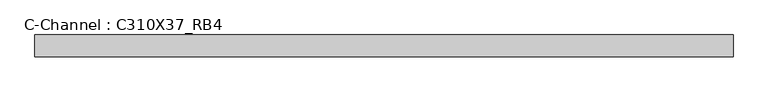
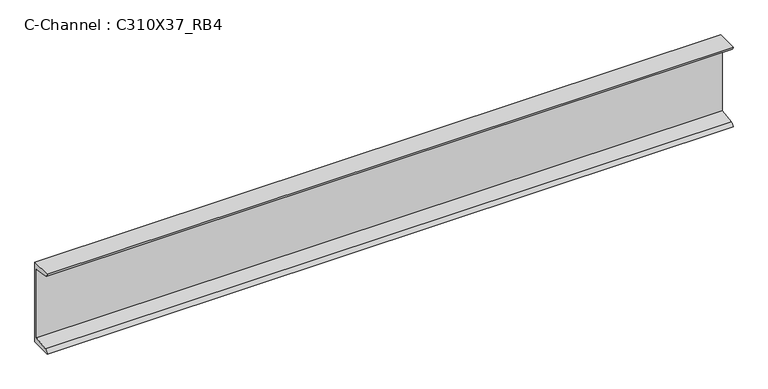
"""IFC4 building model written with IfcOpenShell, lengths in millimetres: beam geometry, C-Channel : C310X37_RB4."""

from ifc_helpers import new_model, si_unit, point, frame, frame_2d, origin, place, context, project, spatial, polyline, circle_curve, trimmed, segment, composite_curve, outline, extrude, source, transform, mapped, element, save


def c_channel_c310x37_rb4_8e0be11c(model_context):
    return source(origin(), model_context, "Body", "SweptSolid", [
        extrude(outline(composite_curve([segment(polyline([(17.1196, 152.4), (17.1196, -152.4), (-60.3504, -152.4)]), True, "CONTINUOUS"), segment(trimmed(circle_curve(frame_2d((-47.625, -152.4)), 12.7254), [point((-60.3504, -152.4))], [point((-47.625, -139.6746))], False, "CARTESIAN"), True, "CONTINUOUS"), segment(polyline([(-47.625, -139.6746), (7.2898, -130.9769501), (7.2898, 130.9769501), (-47.625, 139.6746)]), True, "CONTINUOUS"), segment(trimmed(circle_curve(frame_2d((-47.625, 152.4)), 12.7254), [point((-47.625, 139.6746))], [point((-60.3504, 152.4))], False, "CARTESIAN"), True, "CONTINUOUS"), segment(polyline([(-60.3504, 152.4), (17.1196, 152.4)]), True, "CONTINUOUS")], self_intersect=False)), frame((-1238.3283546, 0.0, 0.0), z_axis=(1.0, 0.0, 0.0), x_axis=(0.0, 1.0, 0.0)), (0.0, 0.0, 1.0), 2479.8217053),
    ])


if __name__ == "__main__":
    model = new_model("IFC4")
    model_context = context("Model", 3, world=origin())
    ifc_project = project(units=[si_unit("LENGTHUNIT", "METRE", prefix="MILLI")], contexts=[model_context])
    site = spatial("IfcSite", under=ifc_project)
    building = spatial("IfcBuilding", under=site)
    placement = place(None, origin())
    c_channel_c310x37_rb4_shape = c_channel_c310x37_rb4_8e0be11c(model_context)
    element("IfcBeam", 1, ObjectType="C-Channel : C310X37_RB4", at=placement, inside=building, context=model_context, shape_type="MappedRepresentation", body=[
        mapped(c_channel_c310x37_rb4_shape, transform((0.0, 0.0, 0.0), x_axis=(1.0, 0.0, 0.0), y_axis=(0.0, 1.0, 0.0), z_axis=(0.0, 0.0, 1.0))),
    ])
    save(model, "model.ifc")

# Revit data of these elements
# Type "C-Channel : C310X37_RB4"
#   Assembly Code = "B10"
#   W = 25
#   Length [instance default] = 1524 mm
#   bf = 77.47 mm
#   d = 304.8 mm
#   tf = 12.725 mm
#   tw = 9.83 mm
#   x = 17.12 mm
#   A = 0.00473547 m²
#   Structural Material [instance default] = Steel ASTM A36
# Element 1 (IfcBeam, "C-Channel : C310X37_RB4")
#   Structural Material = Steel ASTM A992
#   Materials on its faces: "Steel ASTM A992"
# Materials
#   "Steel ASTM A36": class "Metal", colour RGB 199 199 199, transparency 0, Description = "Structural steel, ASTM A36 Grade B, mill finish", Cost = 0
#   "Steel ASTM A992": class "Metal", colour RGB 199 199 199, transparency 0, Description = "Structural steel 50ksi", Cost = 0
